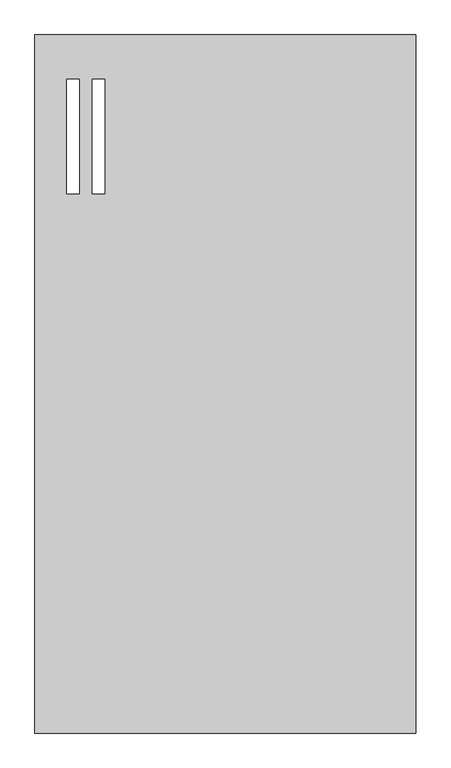
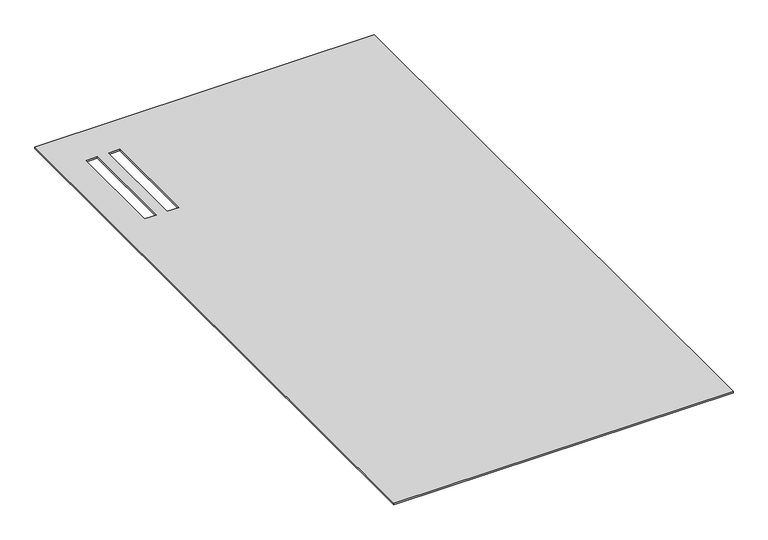
"""IFC4 building model written with IfcOpenShell, lengths in millimetres: proxy geometry, TSP Geyser Electrcical 200L : TSP Geyser Electrcical 200L."""

from ifc_helpers import new_model, si_unit, origin, origin_with_axes, place, context, project, spatial, polyline, outline, extrude, source, transform, mapped, element, save


def electrical_fixtures_ea5495d1(model_context):
    return source(origin(), model_context, "Body", "SweptSolid", [
        extrude(outline(polyline([(-600.0, 600.0), (0.0, 600.0), (0.0, -500.0), (-600.0, -500.0), (-600.0, 600.0)]), holes=[polyline([(-530.0, 530.0), (-550.0, 530.0), (-550.0, 350.0), (-530.0, 350.0), (-530.0, 530.0)]), polyline([(-490.0, 530.0), (-510.0, 530.0), (-510.0, 350.0), (-490.0, 350.0), (-490.0, 530.0)])]), origin_with_axes(), (0.0, 0.0, 1.0), 3.0),
    ])


if __name__ == "__main__":
    model = new_model("IFC4")
    model_context = context("Model", 3, world=origin())
    ifc_project = project(units=[si_unit("LENGTHUNIT", "METRE", prefix="MILLI")], contexts=[model_context])
    site = spatial("IfcSite", under=ifc_project)
    building = spatial("IfcBuilding", under=site)
    placement = place(None, origin())
    electrical_fixtures_shape = electrical_fixtures_ea5495d1(model_context)
    element("IfcBuildingElementProxy", 1, Name="TSP Geyser Electrcical 200L : TSP Geyser Electrcical 200L", ObjectType="TSP Geyser Electrcical 200L : TSP Geyser Electrcical 200L", at=placement, inside=building, context=model_context, shape_type="MappedRepresentation", body=[
        mapped(electrical_fixtures_shape, transform((0.0, 0.0, 0.0), x_axis=(1.0, 0.0, 0.0), y_axis=(0.0, 1.0, 0.0), z_axis=(0.0, 0.0, 1.0))),
    ])
    save(model, "model.ifc")

# Revit data of these elements
# Type "TSP Geyser Electrcical 200L : TSP Geyser Electrcical 200L"
#   Model = "TSP_EGEY200"
#   Default Elevation = 0
# Element 1 (IfcBuildingElementProxy, "TSP Geyser Electrcical 200L : TSP Geyser Electrcical 200L")
#   Materials on its faces: "Aluminum, Anodized Red"
# Materials
#   "Aluminum, Anodized Red": class "Metal", colour RGB 120 120 120, transparency 0, Description = "Anodized aluminum, red", Cost = 0
